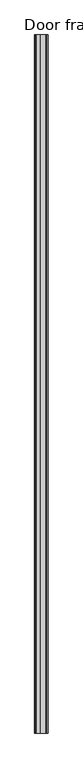
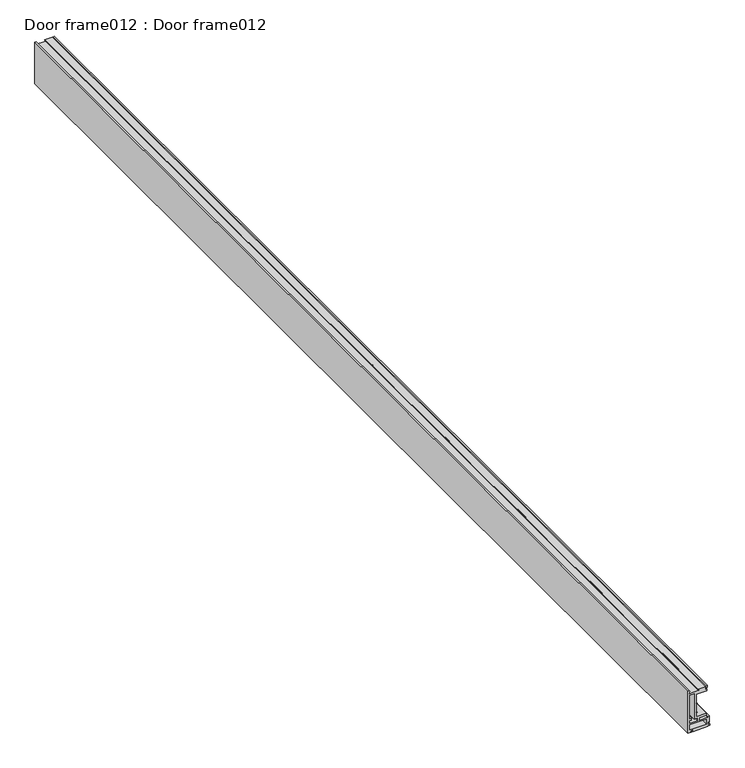
"""IFC4 building model written with IfcOpenShell, lengths in millimetres: proxy geometry, Door frame012 : Door frame012."""

from ifc_helpers import new_model, si_unit, frame, origin, place, context, project, spatial, polyline, outline, extrude, source, transform, mapped, element, save


def door_frame012_door_frame012_2ed3f318(model_context):
    return source(origin(), model_context, "Body", "SweptSolid", [
        extrude(outline(polyline([(36608.9977225, 15539.5084948), (36608.9977225, 15524.517453), (36613.8237225, 15524.517453), (36613.8237225, 15537.3384133), (36616.9987225, 15537.3384133), (36616.9987225, 15519.5076168), (36623.9157731, 15519.5076168), (36624.8727225, 15520.9106887), (36625.8290531, 15519.5076168), (36640.6803935, 15519.5076168), (36641.6367241, 15520.9106887), (36642.5936735, 15519.5076168), (36658.8030324, 15519.5076168), (36658.8030324, 15538.2476818), (36662.4618113, 15538.2476818), (36661.0188583, 15535.7484139), (36666.3421883, 15535.7484139), (36665.4690732, 15539.0049628), (36668.703989, 15539.288472), (36667.561659, 15536.9486127), (36667.7957063, 15535.7484139), (36667.7957063, 15522.1352688), (36666.5824658, 15522.1352688), (36666.5824658, 15523.6520602), (36664.6229889, 15523.6520602), (36664.6229889, 15506.8580308), (36666.7222221, 15506.8580308), (36668.7089205, 15508.0054504), (36669.4492947, 15507.5857589), (36669.4492947, 15504.8264133), (36591.6236909, 15504.8264133), (36591.6236909, 15510.4085802), (36592.8950628, 15510.4085802), (36592.8950628, 15509.5254133), (36594.1652793, 15509.5254133), (36594.1652793, 15514.0974128), (36592.8950628, 15514.0974128), (36592.8950628, 15513.2142459), (36591.6240434, 15513.2142459), (36591.6240434, 15540.1828722), (36593.5561506, 15540.1828722), (36593.5561506, 15541.3652071), (36592.4137824, 15543.7050664), (36595.6486981, 15543.4215572), (36594.775583, 15540.1650084), (36600.1211436, 15540.1650084), (36598.5843732, 15542.6834949), (36610.4200435, 15542.6834949), (36610.4200435, 15539.5084948), (36608.9977225, 15539.5084948)]), holes=[polyline([(36608.9977225, 15508.0061443), (36613.8237225, 15508.0061443), (36613.8237225, 15511.1764133), (36616.9987225, 15511.1764133), (36616.9987225, 15508.0014133), (36661.4479889, 15508.0014133), (36661.4479889, 15516.3326168), (36613.8237225, 15516.3326168), (36613.8237225, 15521.3411443), (36608.9977225, 15521.3411443), (36608.9977225, 15508.0061443)]), polyline([(36605.8183749, 15537.6432186), (36596.3988909, 15537.6432186), (36596.3988909, 15508.0014133), (36605.8183749, 15508.0014133), (36605.8183749, 15537.6432186)])]), frame((0.0, -1052.8906567, 0.0), z_axis=(0.0, 1.0, 0.0), x_axis=(0.0, 0.0, 1.0)), (0.0, 0.0, 1.0), 1999.85),
    ])


if __name__ == "__main__":
    model = new_model("IFC4")
    model_context = context("Model", 3, world=origin())
    ifc_project = project(units=[si_unit("LENGTHUNIT", "METRE", prefix="MILLI")], contexts=[model_context])
    site = spatial("IfcSite", under=ifc_project)
    building = spatial("IfcBuilding", under=site)
    placement = place(None, origin())
    door_frame012_door_frame012_shape = door_frame012_door_frame012_2ed3f318(model_context)
    element("IfcBuildingElementProxy", 1, Name="Door frame012 : Door frame012", ObjectType="Door frame012 : Door frame012", at=placement, inside=building, context=model_context, shape_type="MappedRepresentation", body=[
        mapped(door_frame012_door_frame012_shape, transform((0.0, 0.0, 0.0), x_axis=(1.0, 0.0, 0.0), y_axis=(0.0, 1.0, 0.0), z_axis=(0.0, 0.0, 1.0))),
    ])
    save(model, "model.ifc")

# Revit data of these elements
# Type "Door frame012 : Door frame012"
#   NameOverride = "Door frame012"
# Element 1 (IfcBuildingElementProxy, "Door frame012 : Door frame012")
#   Materials on its faces: "FLEETWOOD SERIES T-3200 SINGLE SWING DOOR FRAME"
# Materials
#   "FLEETWOOD SERIES T-3200 SINGLE SWING DOOR FRAME": class "Unassigned", colour RGB 128 128 128, transparency 0, Cost = 0
